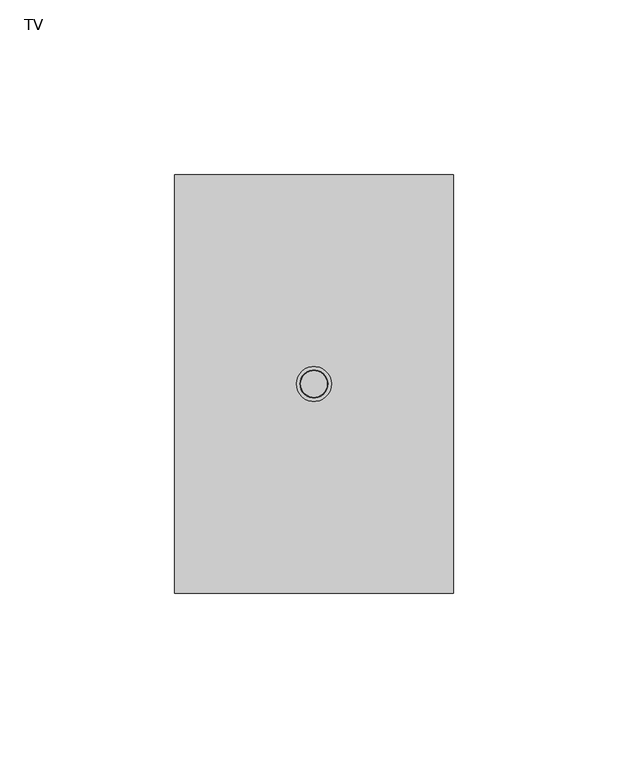
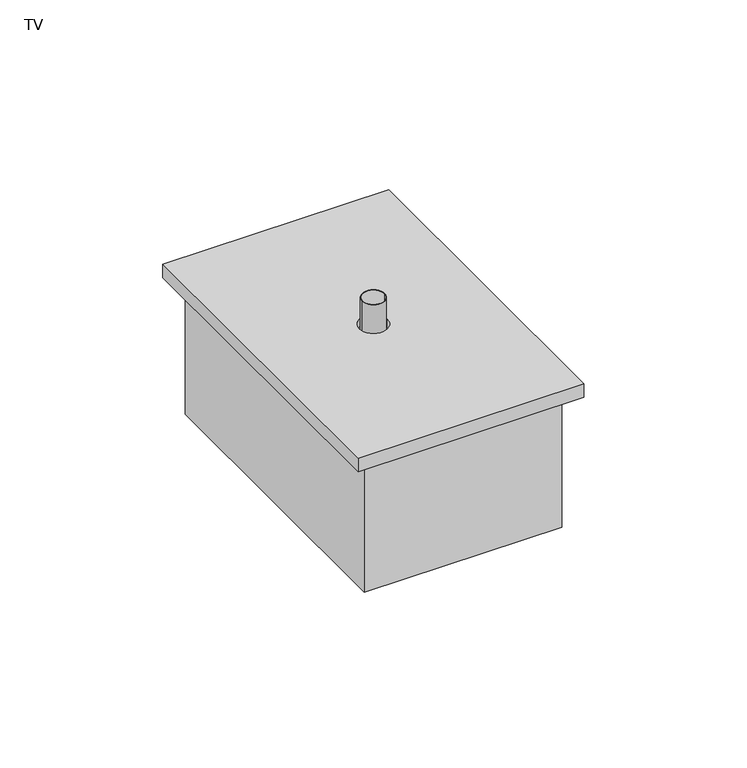
"""IFC4 building model written with IfcOpenShell, lengths in millimetres: proxy geometry, CAIXA VERTICE V7 : TV."""

import ifcopenshell
import ifcopenshell.guid

model = None  # the IFC model being written
_history = None  # IfcOwnerHistory: only IFC2X3 demands one
_inside = {}  # id of a spatial element -> (the spatial element, [elements in it])
_under = {}  # id of a project, library or spatial element -> (it, [spatial elements below it])
_declared = {}  # id of a project -> (the project, [libraries it declares])
_typed = {}  # id of a type object -> (the type object, [elements of that type])
_made_of = {}  # id of a material, layer set ... -> (it, [elements and type objects made of it])


def new_model(schema):
    """Start an empty IFC model of exactly this schema.

    Asked for "IFC4X3", IfcOpenShell would pick the latest addendum, in which some entities
    have other attributes; the version numbers below select the first issue.
    IFC2X3 requires an IfcOwnerHistory on every rooted entity: one is made here for all.
    """
    global model, _history
    if schema == "IFC4X3":
        model = ifcopenshell.file(schema_version=(4, 3, 0, 0))
    else:
        model = ifcopenshell.file(schema=schema)
    _inside.clear()
    _under.clear()
    _declared.clear()
    _typed.clear()
    _made_of.clear()
    _history = None
    if model.schema == "IFC2X3":
        org = make("IfcOrganization", Name="unknown")
        user = make(
            "IfcPersonAndOrganization",
            ThePerson=make("IfcPerson", FamilyName="unknown"),
            TheOrganization=org,
        )
        app = make(
            "IfcApplication",
            ApplicationDeveloper=org,
            Version="unknown",
            ApplicationFullName="unknown",
            ApplicationIdentifier="unknown",
        )
        _history = make(
            "IfcOwnerHistory",
            OwningUser=user,
            OwningApplication=app,
            ChangeAction="ADDED",
            CreationDate=0,
        )
    return model


def make(cls, **values):
    """One entity of the class cls with the attributes given. An attribute that is None is left unset."""
    return model.create_entity(
        cls, **{name: value for name, value in values.items() if value is not None}
    )


def rooted(cls, **values):
    """An entity with a GlobalId (a new one), such as an element, a storey or a relation."""
    return make(cls, GlobalId=ifcopenshell.guid.new(), OwnerHistory=_history, **values)


def si_unit(unit_type, name, prefix=None):
    """IfcSIUnit, for example si_unit("LENGTHUNIT", "METRE", prefix="MILLI")."""
    return make("IfcSIUnit", UnitType=unit_type, Prefix=prefix, Name=name)


def assignment(units):
    """IfcUnitAssignment: the units of a project."""
    return None if units is None else make("IfcUnitAssignment", Units=units)


def point(xyz):
    """IfcCartesianPoint."""
    return None if xyz is None else make("IfcCartesianPoint", Coordinates=xyz)


def direction(xyz):
    """IfcDirection."""
    return None if xyz is None else make("IfcDirection", DirectionRatios=xyz)


def frame(location, z_axis=None, x_axis=None):
    """IfcAxis2Placement3D, a coordinate frame: its origin and axes. An axis left out is left unset."""
    return make(
        "IfcAxis2Placement3D",
        Location=point(location),
        Axis=direction(z_axis),
        RefDirection=direction(x_axis),
    )


def frame_2d(location, x_axis=None):
    """IfcAxis2Placement2D, a coordinate frame in the plane: its origin and x axis."""
    return make(
        "IfcAxis2Placement2D", Location=point(location), RefDirection=direction(x_axis)
    )


def origin():
    """The frame at (0, 0, 0) with its axes left unset."""
    return frame((0.0, 0.0, 0.0))


def origin_with_axes():
    """The frame at (0, 0, 0) with the z axis (0, 0, 1) and the x axis (1, 0, 0) written out."""
    return frame((0.0, 0.0, 0.0), z_axis=(0.0, 0.0, 1.0), x_axis=(1.0, 0.0, 0.0))


def place(relative_to, where):
    """IfcLocalPlacement: puts the frame where relative to a parent placement (None: the world)."""
    return make(
        "IfcLocalPlacement", PlacementRelTo=relative_to, RelativePlacement=where
    )


def context(
    kind, dimensions, precision=None, world=None, true_north=None, identifier=None
):
    """IfcGeometricRepresentationContext, for example the 3D "Model" context."""
    return make(
        "IfcGeometricRepresentationContext",
        ContextIdentifier=identifier,
        ContextType=kind,
        CoordinateSpaceDimension=dimensions,
        Precision=precision,
        WorldCoordinateSystem=world,
        TrueNorth=true_north,
    )


def project(units=None, contexts=None):
    """IfcProject with its units and contexts."""
    return rooted(
        "IfcProject",
        Name="project",
        RepresentationContexts=contexts,
        UnitsInContext=assignment(units),
    )


def spatial(cls, under=None, at=None, **own):
    """A site, building, storey or space (cls), placed at a placement, below another one or the project."""
    s = rooted(cls, ObjectPlacement=at, **own)
    if under is not None:
        _under.setdefault(under.id(), (under, []))[1].append(s)
    return s


def polyline(points):
    """IfcPolyline through the points."""
    return make("IfcPolyline", Points=[point(p) for p in points])


def circle_curve(where, radius):
    """IfcCircle in the frame where."""
    return make("IfcCircle", Position=where, Radius=radius)


def trimmed(basis, trim1, trim2, sense, master):
    """IfcTrimmedCurve: the piece of a basis curve between two trims."""
    return make(
        "IfcTrimmedCurve",
        BasisCurve=basis,
        Trim1=trim1,
        Trim2=trim2,
        SenseAgreement=sense,
        MasterRepresentation=master,
    )


def segment(curve, same_sense, transition):
    """IfcCompositeCurveSegment."""
    return make(
        "IfcCompositeCurveSegment",
        Transition=transition,
        SameSense=same_sense,
        ParentCurve=curve,
    )


def composite_curve(segments, self_intersect=None):
    """IfcCompositeCurve: segments joined end to end."""
    return make("IfcCompositeCurve", Segments=segments, SelfIntersect=self_intersect)


def outline(outer, holes=None, kind="AREA"):
    """IfcArbitraryClosedProfileDef: a profile drawn as a closed curve; with holes, ...WithVoids."""
    if holes is None:
        return make("IfcArbitraryClosedProfileDef", ProfileType=kind, OuterCurve=outer)
    return make(
        "IfcArbitraryProfileDefWithVoids",
        ProfileType=kind,
        OuterCurve=outer,
        InnerCurves=holes,
    )


def extrude(swept, where, along, depth):
    """IfcExtrudedAreaSolid: the profile swept, set in the frame where, extruded along a direction by depth."""
    return make(
        "IfcExtrudedAreaSolid",
        SweptArea=swept,
        Position=where,
        ExtrudedDirection=direction(along),
        Depth=depth,
    )


def faces_of(points, faces, orient=None, outer=None):
    """IfcFace entities. A face is a list of loops; a loop is a list of indices into points, from 0.

    orient and outer hold one flag for each loop. By default every Orientation is true, the
    first loop of a face is its IfcFaceOuterBound and the others are IfcFaceBound.
    """
    made = []
    for i, loops in enumerate(faces):
        bounds = []
        for j, loop in enumerate(loops):
            is_outer = j == 0 if outer is None else outer[i][j]
            bounds.append(
                make(
                    "IfcFaceOuterBound" if is_outer else "IfcFaceBound",
                    Bound=make("IfcPolyLoop", Polygon=[points[k] for k in loop]),
                    Orientation=True if orient is None else orient[i][j],
                )
            )
        made.append(make("IfcFace", Bounds=bounds))
    return made


def faceted_brep(points, faces, orient=None, outer=None, voids=None):
    """IfcFacetedBrep: a solid bounded by flat faces; with voids (closed shells), ...WithVoids."""
    shared = [point(p) for p in points]
    hull = make("IfcClosedShell", CfsFaces=faces_of(shared, faces, orient, outer))
    if voids is None:
        return make("IfcFacetedBrep", Outer=hull)
    return make(
        "IfcFacetedBrepWithVoids",
        Outer=hull,
        Voids=[
            make(cls, CfsFaces=faces_of(shared, fs, o, b)) for cls, fs, o, b in voids
        ],
    )


def shape(context_of_items, identifier, shape_type, items):
    """IfcShapeRepresentation: the items that make up one representation, for example the "Body"."""
    return make(
        "IfcShapeRepresentation",
        ContextOfItems=context_of_items,
        RepresentationIdentifier=identifier,
        RepresentationType=shape_type,
        Items=items,
    )


def source(mapping_origin, context_of_items, identifier, shape_type, items):
    """IfcRepresentationMap: a shape defined once, which mapped items show again and again."""
    return make(
        "IfcRepresentationMap",
        MappingOrigin=mapping_origin,
        MappedRepresentation=shape(context_of_items, identifier, shape_type, items),
    )


def transform(
    local_origin,
    x_axis=None,
    y_axis=None,
    z_axis=None,
    scale=None,
    scale2=None,
    scale3=None,
    uniform=True,
):
    """IfcCartesianTransformationOperator3D, or its non-uniform kind. x_axis, y_axis, z_axis: its Axis1, 2, 3."""
    if uniform:
        return make(
            "IfcCartesianTransformationOperator3D",
            Axis1=direction(x_axis),
            Axis2=direction(y_axis),
            LocalOrigin=point(local_origin),
            Scale=scale,
            Axis3=direction(z_axis),
        )
    return make(
        "IfcCartesianTransformationOperator3DnonUniform",
        Axis1=direction(x_axis),
        Axis2=direction(y_axis),
        LocalOrigin=point(local_origin),
        Scale=scale,
        Axis3=direction(z_axis),
        Scale2=scale2,
        Scale3=scale3,
    )


def mapped(mapping_source, mapping_target):
    """IfcMappedItem: shows the shape of a source again, moved by a transform."""
    return make(
        "IfcMappedItem", MappingSource=mapping_source, MappingTarget=mapping_target
    )


def made_of(thing, what):
    """Note that an element or type object is made of a material, layer set ...; save() writes the relation."""
    if what is not None:
        _made_of.setdefault(what.id(), (what, []))[1].append(thing)
    return thing


def element(
    cls,
    number,
    at=None,
    inside=None,
    cuts=None,
    type_object=None,
    material=None,
    context=None,
    identifier="Body",
    shape_type=None,
    held_by="IfcProductDefinitionShape",
    body=None,
    shapes=None,
    **own,
):
    """One element of the class cls, such as IfcWall. Its Tag is "e" and its number.

    at: its placement. inside: the storey or other place that contains it. cuts: it is an
    opening in that element (IfcRelVoidsElement). A single representation is given by context,
    identifier, shape_type and body (its items); several are given by shapes. held_by: the class
    of the entity that holds the representations. save() writes the other relations.
    """
    e = rooted(cls, Tag="e%d" % number, ObjectPlacement=at, **own)
    if body is not None:
        shapes = [shape(context, identifier, shape_type, body)]
    if shapes is not None:
        e.Representation = make(held_by, Representations=shapes)
    if inside is not None:
        _inside.setdefault(inside.id(), (inside, []))[1].append(e)
    if cuts is not None:
        rooted(
            "IfcRelVoidsElement", RelatingBuildingElement=cuts, RelatedOpeningElement=e
        )
    if type_object is not None:
        _typed.setdefault(type_object.id(), (type_object, []))[1].append(e)
    return made_of(e, material)


def aggregate(whole, parts):
    """IfcRelAggregates: a whole, such as a stair, and the parts it consists of."""
    return rooted("IfcRelAggregates", RelatingObject=whole, RelatedObjects=parts)


def save(model, path):
    """Write the relations noted so far, then the file.

    IfcRelAggregates (storeys below a building ...), IfcRelContainedInSpatialStructure (elements
    in a storey), IfcRelDefinesByType, IfcRelAssociatesMaterial and IfcRelDeclares: one each for
    every whole, place, type object, material and project.
    """
    for whole, parts in _under.values():
        aggregate(whole, parts)
    for where, things in _inside.values():
        rooted(
            "IfcRelContainedInSpatialStructure",
            RelatedElements=things,
            RelatingStructure=where,
        )
    for kind, things in _typed.values():
        rooted("IfcRelDefinesByType", RelatedObjects=things, RelatingType=kind)
    for what, things in _made_of.values():
        rooted("IfcRelAssociatesMaterial", RelatedObjects=things, RelatingMaterial=what)
    for by, libraries in _declared.values():
        rooted("IfcRelDeclares", RelatingContext=by, RelatedDefinitions=libraries)
    model.write(path)


def plane_surface(at):
    """IfcPlane: the flat surface through the origin of the frame at, square to its z axis."""
    return make("IfcPlane", Position=at)


def revolved_surface(curve, axis_point, axis_direction):
    """IfcSurfaceOfRevolution: the curve turned about the line through axis_point along axis_direction."""
    return make(
        "IfcSurfaceOfRevolution",
        SweptCurve=make("IfcArbitraryOpenProfileDef", ProfileType="CURVE", Curve=curve),
        AxisPosition=make("IfcAxis1Placement", Location=point(axis_point), Axis=direction(axis_direction)),
    )


def advanced_brep(points, edges, surfaces, faces):
    """IfcAdvancedBrep: a solid bounded by faces that lie on surfaces and meet in shared edges.

    An edge is (start, end): straight between two places in points (the first is 0);
    or (start, end, curve); or (start, end, curve, False) where it runs against its curve.
    A face is (place in surfaces, loops), or (place, loops, False) where it looks against
    its surface's normal. A loop lists edges by number (the first is 1), with a minus sign
    where the edge is run from its end to its start. The first loop is the outer one.
    """
    corners = [point(p) for p in points]
    vertices = [make("IfcVertexPoint", VertexGeometry=c) for c in corners]
    made = []
    for start, end, *more in edges:
        made.append(
            make(
                "IfcEdgeCurve",
                EdgeStart=vertices[start],
                EdgeEnd=vertices[end],
                EdgeGeometry=more[0] if more else make("IfcPolyline", Points=[corners[start], corners[end]]),
                SameSense=more[1] if len(more) > 1 else True,
            )
        )
    hull = []
    for where, loops, *sense in faces:
        bounds = []
        for j, loop in enumerate(loops):
            ring = [make("IfcOrientedEdge", EdgeElement=made[abs(k) - 1], Orientation=k > 0) for k in loop]
            bounds.append(
                make(
                    "IfcFaceOuterBound" if j == 0 else "IfcFaceBound",
                    Bound=make("IfcEdgeLoop", EdgeList=ring),
                    Orientation=True,
                )
            )
        hull.append(make("IfcAdvancedFace", Bounds=bounds, FaceSurface=surfaces[where], SameSense=sense[0] if sense else True))
    return make("IfcAdvancedBrep", Outer=make("IfcClosedShell", CfsFaces=hull))


def tv_d54fe5a2(model_context):
    return source(origin(), model_context, "Body", "SolidModel", [
        extrude(outline(composite_curve([segment(trimmed(circle_curve(frame_2d((0.0, 1100.0)), 4.0), [point((-4.0, 1100.0))], [point((4.0, 1100.0))], False, "CARTESIAN"), True, "CONTINUOUS"), segment(trimmed(circle_curve(frame_2d((0.0, 1100.0)), 4.0), [point((4.0, 1100.0))], [point((-4.0, 1100.0))], False, "CARTESIAN"), True, "CONTINUOUS")], self_intersect=False), holes=[composite_curve([segment(trimmed(circle_curve(frame_2d((0.0, 1100.0)), 3.8), [point((-3.8, 1100.0))], [point((3.8, 1100.0))], True, "CARTESIAN"), True, "CONTINUOUS"), segment(trimmed(circle_curve(frame_2d((0.0, 1100.0)), 3.8), [point((3.8, 1100.0))], [point((-3.8, 1100.0))], True, "CARTESIAN"), True, "CONTINUOUS")], self_intersect=False)]), origin_with_axes(), (0.0, 0.0, 1.0), 15.0),
        faceted_brep([(33.0, 1047.0, -48.0), (33.0, 1153.0, -48.0), (-33.0, 1153.0, -48.0), (-33.0, 1047.0, -48.0), (35.0, 1155.0, -50.0), (35.0, 1045.0, -50.0), (-35.0, 1045.0, -50.0), (-35.0, 1155.0, -50.0), (-35.0, 1155.0, 0.0), (35.0, 1155.0, 0.0), (-35.0, 1045.0, 0.0), (35.0, 1045.0, 0.0), (33.0, 1153.0, 0.0), (33.0, 1047.0, 0.0), (-33.0, 1047.0, 0.0), (-33.0, 1153.0, 0.0)], [[[0, 1, 2, 3]], [[4, 5, 6, 7]], [[4, 7, 8, 9]], [[8, 7, 6, 10]], [[10, 6, 5, 11]], [[11, 5, 4, 9]], [[9, 8, 10, 11], [12, 13, 14, 15]], [[13, 12, 1, 0]], [[14, 13, 0, 3]], [[15, 14, 3, 2]], [[12, 15, 2, 1]]]),
        advanced_brep(
        [(40.0, 1160.0, 5.0), (-40.0, 1160.0, 5.0), (-40.0, 1040.0, 5.0), (40.0, 1040.0, 5.0), (5.0, 1100.0, 5.0), (-5.0, 1100.0, 5.0), (-40.0, 1160.0, 0.0), (40.0, 1160.0, 0.0), (40.0, 1040.0, 0.0), (-40.0, 1040.0, 0.0), (5.0, 1100.0, 2.0), (-5.0, 1100.0, 2.0)],
        [
            (0, 1),
            (1, 2),
            (2, 3),
            (3, 0),
            (4, 5, circle_curve(frame((0.0, 1100.0, 5.0), z_axis=(0.0, 0.0, -1.0), x_axis=(1.0, 0.0, 0.0)), 5.0)),
            (5, 4, circle_curve(frame((0.0, 1100.0, 5.0), z_axis=(0.0, 0.0, -1.0), x_axis=(1.0, 0.0, 0.0)), 5.0)),
            (6, 7),
            (7, 8),
            (8, 9),
            (9, 6),
            (0, 7),
            (6, 1),
            (9, 2),
            (8, 3),
            (10, 11, circle_curve(frame((0.0, 1100.0, 2.0), z_axis=(0.0, 0.0, -1.0), x_axis=(1.0, 0.0, 0.0)), 5.0)),
            (11, 5),
            (4, 10),
            (10, 11, circle_curve(frame((0.0, 1100.0, 2.0), z_axis=(0.0, 0.0, 1.0), x_axis=(1.0, 0.0, 0.0)), 5.0)),
        ],
        [
            plane_surface(frame((-60.0, 1160.0, 5.0), z_axis=(0.0, 0.0, 1.0), x_axis=(-1.0, 0.0, 0.0))),
            plane_surface(frame((-60.0, 1160.0, 0.0), z_axis=(0.0, 0.0, -1.0), x_axis=(1.0, 0.0, 0.0))),
            plane_surface(frame((40.0, 1160.0, 5.0), z_axis=(0.0, 1.0, 0.0), x_axis=(0.0, 0.0, -1.0))),
            plane_surface(frame((-40.0, 1160.0, 5.0), z_axis=(-1.0, 0.0, 0.0), x_axis=(0.0, 0.0, -1.0))),
            plane_surface(frame((-40.0, 1040.0, 5.0), z_axis=(0.0, -1.0, 0.0), x_axis=(0.0, 0.0, -1.0))),
            plane_surface(frame((40.0, 1040.0, 5.0), z_axis=(1.0, 0.0, 0.0), x_axis=(0.0, 0.0, -1.0))),
            revolved_surface(polyline([(5.0, 1100.0, 5.0), (5.0, 1100.0, 2.0)]), (0.0, 1100.0, 2.0), (0.0, 0.0, 1.0)),
            plane_surface(frame((5.0, 1100.0, 2.0), z_axis=(0.0, 0.0, 1.0), x_axis=(0.0, -1.0, 0.0))),
        ],
        [
            (0, [[1, 2, 3, 4], [5, 6]]),
            (1, [[7, 8, 9, 10]]),
            (2, [[-1, 11, -7, 12]]),
            (3, [[-2, -12, -10, 13]]),
            (4, [[-3, -13, -9, 14]]),
            (5, [[-4, -14, -8, -11]]),
            (6, [[15, 16, -5, 17]]),
            (7, [[-15, 18]]),
            (6, [[-18, -17, -6, -16]]),
        ],
    ),
    ])


if __name__ == "__main__":
    model = new_model("IFC4")
    model_context = context("Model", 3, world=origin())
    ifc_project = project(units=[si_unit("LENGTHUNIT", "METRE", prefix="MILLI")], contexts=[model_context])
    site = spatial("IfcSite", under=ifc_project)
    building = spatial("IfcBuilding", under=site)
    placement = place(None, origin())
    tv_shape = tv_d54fe5a2(model_context)
    element("IfcBuildingElementProxy", 1, Name="CAIXA VERTICE V7 : TV", ObjectType="CAIXA VERTICE V7 : TV", at=placement, inside=building, context=model_context, shape_type="MappedRepresentation", body=[
        mapped(tv_shape, transform((0.0, 0.0, 0.0), x_axis=(1.0, 0.0, 0.0), y_axis=(0.0, 1.0, 0.0), z_axis=(0.0, 0.0, 1.0))),
    ])
    save(model, "model.ifc")

# Revit data of these elements
# Type "CAIXA VERTICE V7 : TV"
#   URL = "www.facebook.com/verticetreinamentos"
#   SEÇÃO [instance default] = ""
#   Rotação [instance default] = 0.00°
#   LARGURA DA TAMPA = 0.08 m
#   BORDA = 0.01 m
#   ALTURA DE INSTALAÇÃO [instance default] = 1.10 m
#   Distância Anotação [instance default] = 0.0015 m
#   ALTURA DA TAMPA = 0.12 m
#   Vertical [instance default] = yes
#   VER SEÇÃO [instance default] = no
#   SHADE ESQ [instance default] = no
#   SHADE DIR [instance default] = yes
#   HORIZONTAL [instance default] = no
#   ANDAR COM A LEGENDA [instance default] = 0
#   Material Tampa [instance default] = Plástico, branco opaco
#   Caixa = element 1798535
#   Anotação = element 1798534
#   Default Elevation = 0
# Element 1 (IfcBuildingElementProxy, "CAIXA VERTICE V7 : TV")
#   Materials on its faces: "Plástico, branco opaco"
# Materials
#   "Plástico, branco opaco": class "Plástico", colour RGB 120 120 120, transparency 0, Description = "Plastic, generic, opaque white", Cost = 0
